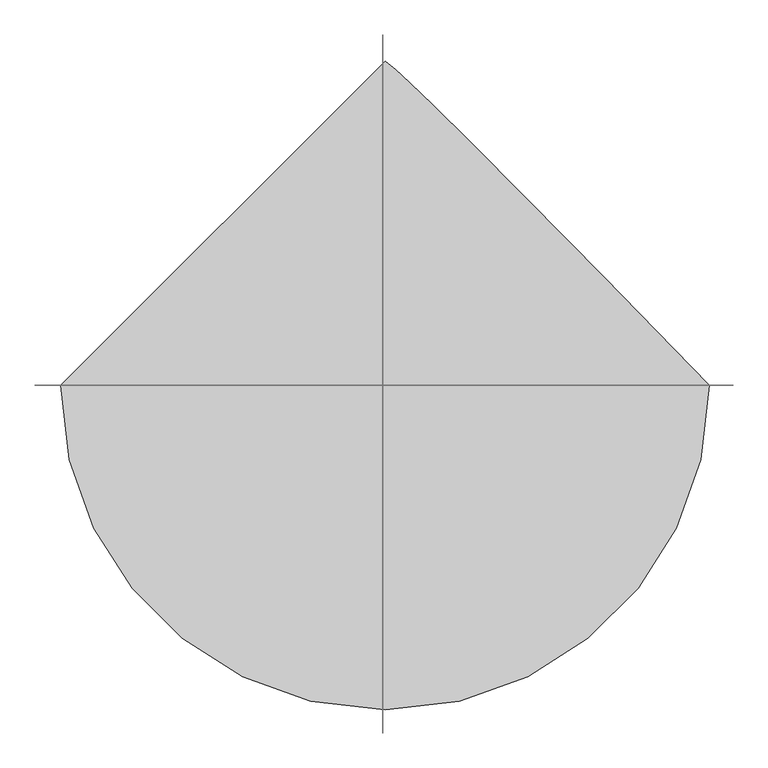
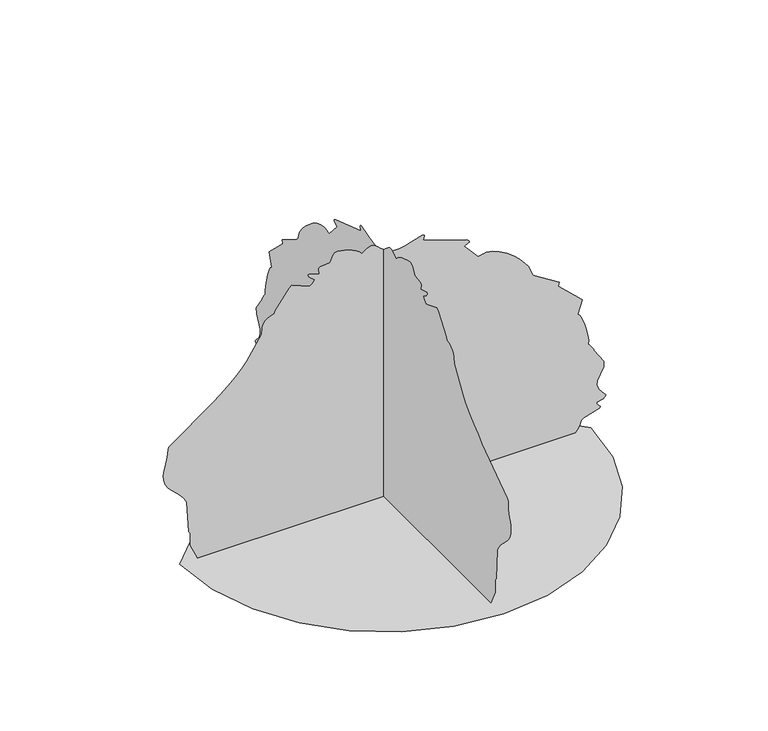
"""IFC4 building model written with IfcOpenShell, lengths in millimetres: proxy geometry, holly 26750 : holly 26750."""

import ifcopenshell
import ifcopenshell.guid

model = None  # the IFC model being written
_history = None  # IfcOwnerHistory: only IFC2X3 demands one
_inside = {}  # id of a spatial element -> (the spatial element, [elements in it])
_under = {}  # id of a project, library or spatial element -> (it, [spatial elements below it])
_declared = {}  # id of a project -> (the project, [libraries it declares])
_typed = {}  # id of a type object -> (the type object, [elements of that type])
_made_of = {}  # id of a material, layer set ... -> (it, [elements and type objects made of it])


def new_model(schema):
    """Start an empty IFC model of exactly this schema.

    Asked for "IFC4X3", IfcOpenShell would pick the latest addendum, in which some entities
    have other attributes; the version numbers below select the first issue.
    IFC2X3 requires an IfcOwnerHistory on every rooted entity: one is made here for all.
    """
    global model, _history
    if schema == "IFC4X3":
        model = ifcopenshell.file(schema_version=(4, 3, 0, 0))
    else:
        model = ifcopenshell.file(schema=schema)
    _inside.clear()
    _under.clear()
    _declared.clear()
    _typed.clear()
    _made_of.clear()
    _history = None
    if model.schema == "IFC2X3":
        org = make("IfcOrganization", Name="unknown")
        user = make(
            "IfcPersonAndOrganization",
            ThePerson=make("IfcPerson", FamilyName="unknown"),
            TheOrganization=org,
        )
        app = make(
            "IfcApplication",
            ApplicationDeveloper=org,
            Version="unknown",
            ApplicationFullName="unknown",
            ApplicationIdentifier="unknown",
        )
        _history = make(
            "IfcOwnerHistory",
            OwningUser=user,
            OwningApplication=app,
            ChangeAction="ADDED",
            CreationDate=0,
        )
    return model


def make(cls, **values):
    """One entity of the class cls with the attributes given. An attribute that is None is left unset."""
    return model.create_entity(
        cls, **{name: value for name, value in values.items() if value is not None}
    )


def rooted(cls, **values):
    """An entity with a GlobalId (a new one), such as an element, a storey or a relation."""
    return make(cls, GlobalId=ifcopenshell.guid.new(), OwnerHistory=_history, **values)


def si_unit(unit_type, name, prefix=None):
    """IfcSIUnit, for example si_unit("LENGTHUNIT", "METRE", prefix="MILLI")."""
    return make("IfcSIUnit", UnitType=unit_type, Prefix=prefix, Name=name)


def assignment(units):
    """IfcUnitAssignment: the units of a project."""
    return None if units is None else make("IfcUnitAssignment", Units=units)


def point(xyz):
    """IfcCartesianPoint."""
    return None if xyz is None else make("IfcCartesianPoint", Coordinates=xyz)


def direction(xyz):
    """IfcDirection."""
    return None if xyz is None else make("IfcDirection", DirectionRatios=xyz)


def frame(location, z_axis=None, x_axis=None):
    """IfcAxis2Placement3D, a coordinate frame: its origin and axes. An axis left out is left unset."""
    return make(
        "IfcAxis2Placement3D",
        Location=point(location),
        Axis=direction(z_axis),
        RefDirection=direction(x_axis),
    )


def origin():
    """The frame at (0, 0, 0) with its axes left unset."""
    return frame((0.0, 0.0, 0.0))


def place(relative_to, where):
    """IfcLocalPlacement: puts the frame where relative to a parent placement (None: the world)."""
    return make(
        "IfcLocalPlacement", PlacementRelTo=relative_to, RelativePlacement=where
    )


def context(
    kind, dimensions, precision=None, world=None, true_north=None, identifier=None
):
    """IfcGeometricRepresentationContext, for example the 3D "Model" context."""
    return make(
        "IfcGeometricRepresentationContext",
        ContextIdentifier=identifier,
        ContextType=kind,
        CoordinateSpaceDimension=dimensions,
        Precision=precision,
        WorldCoordinateSystem=world,
        TrueNorth=true_north,
    )


def project(units=None, contexts=None):
    """IfcProject with its units and contexts."""
    return rooted(
        "IfcProject",
        Name="project",
        RepresentationContexts=contexts,
        UnitsInContext=assignment(units),
    )


def spatial(cls, under=None, at=None, **own):
    """A site, building, storey or space (cls), placed at a placement, below another one or the project."""
    s = rooted(cls, ObjectPlacement=at, **own)
    if under is not None:
        _under.setdefault(under.id(), (under, []))[1].append(s)
    return s


def point_list(points):
    """IfcCartesianPointList2D or 3D."""
    cls = (
        "IfcCartesianPointList2D" if len(points[0]) == 2 else "IfcCartesianPointList3D"
    )
    return make(cls, CoordList=points)


def triangles(points, corners, closed=None, point_numbers=None):
    """IfcTriangulatedFaceSet: each triangle names its three corners, points numbered from 1."""
    return make(
        "IfcTriangulatedFaceSet",
        Coordinates=point_list(points),
        Closed=closed,
        CoordIndex=corners,
        PnIndex=point_numbers,
    )


def shape(context_of_items, identifier, shape_type, items):
    """IfcShapeRepresentation: the items that make up one representation, for example the "Body"."""
    return make(
        "IfcShapeRepresentation",
        ContextOfItems=context_of_items,
        RepresentationIdentifier=identifier,
        RepresentationType=shape_type,
        Items=items,
    )


def source(mapping_origin, context_of_items, identifier, shape_type, items):
    """IfcRepresentationMap: a shape defined once, which mapped items show again and again."""
    return make(
        "IfcRepresentationMap",
        MappingOrigin=mapping_origin,
        MappedRepresentation=shape(context_of_items, identifier, shape_type, items),
    )


def transform(
    local_origin,
    x_axis=None,
    y_axis=None,
    z_axis=None,
    scale=None,
    scale2=None,
    scale3=None,
    uniform=True,
):
    """IfcCartesianTransformationOperator3D, or its non-uniform kind. x_axis, y_axis, z_axis: its Axis1, 2, 3."""
    if uniform:
        return make(
            "IfcCartesianTransformationOperator3D",
            Axis1=direction(x_axis),
            Axis2=direction(y_axis),
            LocalOrigin=point(local_origin),
            Scale=scale,
            Axis3=direction(z_axis),
        )
    return make(
        "IfcCartesianTransformationOperator3DnonUniform",
        Axis1=direction(x_axis),
        Axis2=direction(y_axis),
        LocalOrigin=point(local_origin),
        Scale=scale,
        Axis3=direction(z_axis),
        Scale2=scale2,
        Scale3=scale3,
    )


def mapped(mapping_source, mapping_target):
    """IfcMappedItem: shows the shape of a source again, moved by a transform."""
    return make(
        "IfcMappedItem", MappingSource=mapping_source, MappingTarget=mapping_target
    )


def made_of(thing, what):
    """Note that an element or type object is made of a material, layer set ...; save() writes the relation."""
    if what is not None:
        _made_of.setdefault(what.id(), (what, []))[1].append(thing)
    return thing


def element(
    cls,
    number,
    at=None,
    inside=None,
    cuts=None,
    type_object=None,
    material=None,
    context=None,
    identifier="Body",
    shape_type=None,
    held_by="IfcProductDefinitionShape",
    body=None,
    shapes=None,
    **own,
):
    """One element of the class cls, such as IfcWall. Its Tag is "e" and its number.

    at: its placement. inside: the storey or other place that contains it. cuts: it is an
    opening in that element (IfcRelVoidsElement). A single representation is given by context,
    identifier, shape_type and body (its items); several are given by shapes. held_by: the class
    of the entity that holds the representations. save() writes the other relations.
    """
    e = rooted(cls, Tag="e%d" % number, ObjectPlacement=at, **own)
    if body is not None:
        shapes = [shape(context, identifier, shape_type, body)]
    if shapes is not None:
        e.Representation = make(held_by, Representations=shapes)
    if inside is not None:
        _inside.setdefault(inside.id(), (inside, []))[1].append(e)
    if cuts is not None:
        rooted(
            "IfcRelVoidsElement", RelatingBuildingElement=cuts, RelatedOpeningElement=e
        )
    if type_object is not None:
        _typed.setdefault(type_object.id(), (type_object, []))[1].append(e)
    return made_of(e, material)


def aggregate(whole, parts):
    """IfcRelAggregates: a whole, such as a stair, and the parts it consists of."""
    return rooted("IfcRelAggregates", RelatingObject=whole, RelatedObjects=parts)


def save(model, path):
    """Write the relations noted so far, then the file.

    IfcRelAggregates (storeys below a building ...), IfcRelContainedInSpatialStructure (elements
    in a storey), IfcRelDefinesByType, IfcRelAssociatesMaterial and IfcRelDeclares: one each for
    every whole, place, type object, material and project.
    """
    for whole, parts in _under.values():
        aggregate(whole, parts)
    for where, things in _inside.values():
        rooted(
            "IfcRelContainedInSpatialStructure",
            RelatedElements=things,
            RelatingStructure=where,
        )
    for kind, things in _typed.values():
        rooted("IfcRelDefinesByType", RelatedObjects=things, RelatingType=kind)
    for what, things in _made_of.values():
        rooted("IfcRelAssociatesMaterial", RelatedObjects=things, RelatingMaterial=what)
    for by, libraries in _declared.values():
        rooted("IfcRelDeclares", RelatingContext=by, RelatedDefinitions=libraries)
    model.write(path)


def entourage_c51d7213(model_context):
    return source(origin(), model_context, "Body", "Tessellation", [
        triangles([(-948.1489574, 0.0, 0.0001584), (-923.0842083, -217.2530545, 0.0001584), (-851.6949612, -416.7657311, 0.0001584), (-739.7012884, -592.8207553, 0.0001584), (-592.8207553, -739.7012884, 0.0001584), (-416.7657311, -851.6949612, 0.0001584), (-217.2530545, -923.0816648, 0.0001584), (4.14e-05, -948.1489574, 0.0001584), (217.2530545, -923.0842083, 0.0001584), (416.7657311, -851.6949612, 0.0001584), (592.8207553, -739.7012884, 0.0001584), (739.7012884, -592.8207553, 0.0001584), (851.6949612, -416.7657311, 0.0001584), (923.0816648, -217.2530545, 0.0001584), (948.1489574, 8.29e-05, 0.0001584), (640.0215443, 316.0623576, 0.0001584), (411.5917374, 548.7669763, 0.0001584), (249.5753185, 712.0026157, 0.0001584), (140.6913579, 819.6655935, 0.0001584), (71.6559369, 885.64972, 0.0001584), (29.1863771, 923.8462257, 0.0001584), (-0.0001243, 948.1489574, 0.0001584), (-7.5086714, -195.1763861, 1267.2389282), (-7.5086714, -179.2483067, 1263.2994884), (-7.5086714, -162.0304078, 1257.8307816), (-7.5086714, -144.4787539, 1250.7569401), (-7.5086714, -127.5514259, 1242.0092182), (-7.5086714, -112.2047518, 1231.5139286), (-7.5086714, -99.3960405, 1219.1973839), (-7.5086714, -96.3241623, 1220.6731659), (-7.5086714, -91.1522123, 1224.4323841), (-7.5086714, -84.5334848, 1229.4921043), (-7.5086714, -77.1194751, 1234.8564571), (-7.5086714, -69.5642495, 1239.5377121), (-7.5086714, -62.5195578, 1242.5399998), (-7.5086714, -56.6381899, 1242.880386), (-7.5086714, -48.1497636, 1241.0642178), (-7.5086714, -38.0075433, 1235.3112259), (-7.5086714, -26.6616175, 1226.6954727), (-7.5086714, -14.5605495, 1216.2942181), (-7.5086714, -2.1549868, 1205.1816696), (-7.5086714, 10.1063292, 1194.4323984), (-7.5086714, 21.7735642, 1185.1233009), (-7.5086714, 44.9310738, 1181.1406225), (-7.5086714, 71.2939859, 1182.9871668), (-7.5086714, 98.7844045, 1188.6996088), (-7.5086714, 125.3246087, 1196.3018337), (-7.5086714, 178.4657237, 1210.777331), (-7.5086714, 184.0044481, 1210.1194496), (-7.5086714, 186.6691655, 1206.9444254), (-7.5086714, 187.1967314, 1202.1768385), (-7.5086714, 182.6755321, 1185.5170269), (-7.5086714, 383.1462716, 1117.5161631), (-7.5086714, 393.1767277, 1109.7361147), (-7.5086714, 395.0157143, 1105.6136919), (-7.5086714, 393.8879488, 1102.1694254), (-7.5086714, 390.6062814, 1099.2180067), (-7.5086714, 372.1277581, 1088.6871088), (-7.5086714, 435.2772466, 1017.1175674), (-7.5086714, 437.7283324, 1017.437606), (-7.5086714, 442.2698793, 1018.3037596), (-7.5086714, 448.2439333, 1019.5610229), (-7.5086714, 454.9825481, 1021.0621668), (-7.5086714, 461.822792, 1022.6598164), (-7.5086714, 468.1067471, 1024.2016554), (-7.5086714, 473.166431, 1025.537693), (-7.5086714, 502.5059555, 1020.5592905), (-7.5086714, 534.2381756, 1007.0464525), (-7.5086714, 566.6435014, 987.1252121), (-7.5086714, 598.0048865, 962.9266891), (-7.5086714, 626.6103716, 936.5792421), (-7.5086714, 650.7352798, 910.2089767), (-7.5086714, 668.6702316, 885.9468676), (-7.5086714, 686.5644882, 838.1898262), (-7.5086714, 809.9704004, 760.305772), (-7.5086714, 805.7591022, 743.4655935), (-7.5086714, 915.2203714, 638.2130791), (-7.5086714, 894.1714382, 575.0635906), (-7.5086714, 903.617664, 567.5579078), (-7.5086714, 914.1053232, 547.8068604), (-7.5086714, 924.5625338, 519.9684434), (-7.5086714, 933.9198841, 488.2006877), (-7.5086714, 941.1080355, 456.6564285), (-7.5086714, 945.0552509, 429.4962041), (-7.5086714, 944.6894302, 410.8729222), (-7.5086714, 947.6840876, 408.4091191), (-7.5086714, 951.631303, 403.9311221), (-7.5086714, 956.0813948, 398.0789357), (-7.5086714, 960.5872971, 391.4952533), (-7.5086714, 964.7020895, 384.820152), (-7.5086714, 967.971076, 378.6987597), (-7.5086714, 969.9497343, 373.7711535), (-7.5086714, 1015.9974323, 304.568855), (-7.5086714, 1014.0136871, 276.7279126), (-7.5086714, 984.4354053, 218.9253907), (-7.5086714, 983.4092325, 198.3142941), (-7.5086714, 995.1541552, 172.0712739), (-7.5086714, 1024.6817133, 137.2212117), (-7.5086714, 1022.9417759, 130.8493623), (-7.5086714, 1018.3139334, 126.0055809), (-7.5086714, 1011.6743677, 122.4462869), (-7.5086714, 982.5811581, 116.1709614), (-7.5086714, 982.5024565, 110.3304839), (-7.5086714, 984.7630743, 105.408982), (-7.5086714, 999.0657623, 90.4069817), (-7.5086714, 999.4214092, 86.700867), (-7.5086714, 994.9103474, 81.6175654), (-7.5086714, 922.3882479, 60.3801172), (-7.5086714, 911.0090733, 53.020719), (-7.5086714, 909.9524517, 45.2163171), (-7.5086714, 907.5597198, 37.5411996), (-7.5086714, 904.0596428, 29.9740312), (-7.5086714, 899.6679777, 22.4928926), (-7.5086714, 894.6082575, 15.0766517), (-7.5086714, 889.1066311, 7.7034389), (-7.5086714, 883.3814718, 0.3517747), (-7.5086714, -857.0696331, 0.0), (-7.5086714, -890.8821041, 74.070715), (-7.5086714, -890.8821041, 133.011158), (-7.5086714, -897.8544256, 142.0888652), (-7.5086714, -906.9323599, 288.2569691), (-7.5086714, -918.2785423, 310.329568), (-7.5086714, -934.7885084, 330.547956), (-7.5086714, -954.1814381, 349.7579753), (-7.5086714, -974.171279, 368.8105187), (-7.5086714, -992.4846233, 388.5513923), (-7.5086714, -1006.8356369, 409.831525), (-7.5086714, -1014.945825, 433.5017735), (-7.5086714, -1016.3835279, 454.0351496), (-7.5086714, -1014.4251446, 473.0826061), (-7.5086714, -1010.2722731, 490.9768991), (-7.5086714, -1005.1338512, 508.0558711), (-7.5086714, -996.7289864, 541.0987307), (-7.5086714, -993.7038076, 576.6841312), (-7.5086714, -989.7007816, 586.0592494), (-7.5086714, -986.7239285, 589.1733035), (-7.5086714, -784.7202702, 733.315777), (-7.5086714, -753.8211388, 759.3609169), (-7.5086714, -719.0663561, 789.2566938), (-7.5086714, -684.3724709, 820.8568726), (-7.5086714, -653.6486195, 852.0099129), (-7.5086714, -630.8089525, 880.5697248), (-7.5086714, -562.4982239, 987.6459652), (-7.5086714, -559.6966144, 1020.7294109), (-7.5086714, -555.292232, 1034.4301735), (-7.5086714, -548.0761027, 1046.0812065), (-7.5086714, -537.4512789, 1055.5756851), (-7.5086714, -522.8132552, 1062.7994448), (-7.5086714, -503.5575265, 1067.6381756), (-7.5086714, -500.3495101, 1081.6894255), (-7.5086714, -435.3305863, 1167.4931997), (-7.5086714, -423.5678596, 1177.0969013), (-7.5086714, -339.3668581, 1143.4165443), (-7.5086714, -336.5372706, 1144.8643484), (-7.5086714, -333.0320704, 1147.7802315), (-7.5086714, -329.2195487, 1151.7172005), (-7.5086714, -318.3178522, 1168.6768484), (-7.5086714, -338.9502774, 1184.7296476), (-7.5086714, -344.6017857, 1191.1278763), (-7.5086714, -347.962191, 1197.2136967), (-7.5086714, -347.7869473, 1202.3572054), (-7.5086714, -343.1539816, 1204.0539042), (-7.5086714, -297.2663574, 1189.7283251), (-7.5086714, -299.3516952, 1212.9287258), (-7.5086714, -298.767483, 1216.5431128), (-7.5086714, -297.2663574, 1219.1973839), (-7.5086714, -292.6613332, 1221.3539383), (-7.5086714, -249.2443431, 1226.9900768), (-7.5086714, -246.747021, 1227.6175095), (-7.5086714, -231.2268564, 1258.3413609), (-7.5086714, -224.3381235, 1265.7124226), (-7.5086714, -216.7902557, 1269.9999516), (-7.5086714, -208.8568192, 1269.717992), (-202.6848849, -7.94e-05, 1267.2389282), (-186.7567873, -7.9e-05, 1263.2994884), (-169.5388885, -7.87e-05, 1257.8307816), (-151.9872436, -7.84e-05, 1250.7569401), (-135.0599247, -7.8e-05, 1242.0092182), (-119.7134959, -7.75e-05, 1231.5139286), (-106.9047846, -7.68e-05, 1219.1973839), (-103.8329063, -7.69e-05, 1220.6731659), (-98.6609655, -7.7e-05, 1224.4323841), (-92.0419745, -7.73e-05, 1229.4921043), (-84.6279739, -7.75e-05, 1234.8564571), (-77.0729936, -7.78e-05, 1239.5377121), (-70.0280521, -7.8e-05, 1242.5399998), (-64.1469339, -7.83e-05, 1242.880386), (-55.6582578, -7.75e-05, 1241.0642178), (-45.5160353, -7.69e-05, 1235.3112259), (-34.1701118, -7.64e-05, 1226.6954727), (-22.0691448, -7.6e-05, 1216.2942181), (-9.6635817, -7.56e-05, 1205.1816696), (2.5977342, -7.53e-05, 1194.4323984), (14.26497, -7.48e-05, 1185.1233009), (37.4223274, -7.46e-05, 1181.1406225), (63.7852418, -7.46e-05, 1182.9871668), (91.2759148, -7.49e-05, 1188.6996088), (117.816119, -7.54e-05, 1196.3018337), (170.9569705, -7.63e-05, 1210.777331), (176.4956949, -7.62e-05, 1210.1194496), (179.1604124, -7.6e-05, 1206.9444254), (179.6879783, -7.57e-05, 1202.1768385), (175.1670333, -7.48e-05, 1185.5170269), (375.6380453, -7.06e-05, 1117.5161631), (385.6685014, -7.03e-05, 1109.7361147), (387.5074516, -7.02e-05, 1105.6136919), (386.3797225, -7e-05, 1102.1694254), (383.0980187, -6.98e-05, 1099.2180067), (364.6195318, -6.91e-05, 1088.6871088), (427.7690203, -6.48e-05, 1017.1175674), (430.2201061, -6.48e-05, 1017.437606), (434.7616167, -6.49e-05, 1018.3037596), (440.735707, -6.5e-05, 1019.5610229), (447.4743218, -6.5e-05, 1021.0621668), (454.3145293, -6.51e-05, 1022.6598164), (460.5984844, -6.52e-05, 1024.2016554), (465.6581683, -6.53e-05, 1025.537693), (494.9977292, -6.5e-05, 1020.5592905), (526.7299493, -6.42e-05, 1007.0464525), (559.1352751, -6.3e-05, 987.1252121), (590.4966239, -6.16e-05, 962.9266891), (619.0995655, -6e-05, 936.5792421), (643.2270172, -5.84e-05, 910.2089767), (661.161969, -5.7e-05, 885.9468676), (679.0537548, -5.41e-05, 838.1898262), (802.4621378, -4.95e-05, 760.305772), (798.2508396, -4.85e-05, 743.4655935), (907.7121815, -4.22e-05, 638.2156225), (886.6606321, -3.85e-05, 575.0635906), (896.1094013, -3.8e-05, 567.5579078), (906.5970606, -3.68e-05, 547.8068604), (917.0542711, -3.52e-05, 519.9684434), (926.4116215, -3.33e-05, 488.2006877), (933.5973021, -3.14e-05, 456.6564285), (937.5444448, -2.98e-05, 429.4962041), (937.1812403, -2.87e-05, 410.8729222), (940.1758976, -2.85e-05, 408.4091191), (944.1230404, -2.83e-05, 403.9311221), (948.5731321, -2.79e-05, 398.0789357), (953.0791071, -2.75e-05, 391.4952533), (957.1913561, -2.71e-05, 384.820152), (960.462886, -2.68e-05, 378.6987597), (962.4415443, -2.65e-05, 373.7711535), (1008.4891697, -2.23e-05, 304.568855), (1006.5054245, -2.07e-05, 276.7279126), (976.9271427, -1.72e-05, 218.9253907), (975.9009699, -1.6e-05, 198.3142941), (987.6459652, -1.44e-05, 172.0712739), (1017.1734507, -1.24e-05, 137.2212117), (1015.4335133, -1.2e-05, 130.8493623), (1010.8056707, -1.17e-05, 126.0058353), (1004.1661051, -1.15e-05, 122.4462869), (975.0729681, -1.11e-05, 116.1712157), (974.9941938, -1.11e-05, 110.3304839), (977.2548117, -1.08e-05, 105.408982), (991.5575724, -9.4e-06, 90.407236), (991.9131466, -9.3e-06, 86.700867), (987.4020847, -9.1e-06, 81.6175654), (914.8800579, -7.5e-06, 60.3801172), (903.5008106, -7.3e-06, 53.020719), (902.4441891, -7.5e-06, 45.2163171), (900.0515299, -7.5e-06, 37.5411996), (896.5488367, -7.3e-06, 29.9740312), (892.1597151, -6.9e-06, 22.4929448), (887.1000675, -6.5e-06, 15.0767278), (881.5984411, -6e-06, 7.7034894), (875.8732819, -5.5e-06, 0.3518408), (-864.5778957, -4.1e-06, 6.72e-05), (-898.3903667, -8.6e-06, 74.0709693), (-898.3903667, -1.21e-05, 133.011158), (-905.3626156, -1.26e-05, 142.0888652), (-914.4406225, -2.14e-05, 288.2569691), (-925.7893484, -2.27e-05, 310.3321115), (-942.296771, -2.39e-05, 330.547956), (-961.6897007, -2.5e-05, 349.7579753), (-981.6820124, -2.62e-05, 368.8105187), (-999.992886, -2.73e-05, 388.5513923), (-1014.3438995, -2.86e-05, 409.831525), (-1022.4540876, -3e-05, 433.5017735), (-1023.8917179, -3.12e-05, 454.0351496), (-1021.9334072, -3.24e-05, 473.0826061), (-1017.7805357, -3.34e-05, 490.9768991), (-1012.6421139, -3.45e-05, 508.0558711), (-1004.237249, -3.64e-05, 541.0987307), (-1001.2146137, -3.86e-05, 576.6841312), (-997.2090443, -3.92e-05, 586.0592494), (-994.2347345, -3.94e-05, 589.1733035), (-792.2285328, -4.83e-05, 733.315777), (-761.3294014, -5.01e-05, 759.3609169), (-726.5746187, -5.21e-05, 789.2566938), (-691.8807335, -5.41e-05, 820.8568726), (-661.1568821, -5.59e-05, 852.0099129), (-638.3172152, -5.74e-05, 880.5697248), (-570.0064502, -6.3e-05, 987.6459652), (-567.2048407, -6.5e-05, 1020.7294109), (-562.8004947, -6.58e-05, 1034.4301735), (-555.584329, -6.65e-05, 1046.0812065), (-544.9595052, -6.71e-05, 1055.5756851), (-530.3215178, -6.75e-05, 1062.7994448), (-511.0682962, -6.78e-05, 1067.6381756), (-507.8577364, -6.87e-05, 1081.6894255), (-442.8413561, -7.38e-05, 1167.4931997), (-431.0760859, -7.43e-05, 1177.0969013), (-346.8750844, -7.23e-05, 1143.4165443), (-344.0455333, -7.24e-05, 1144.8643484), (-340.540333, -7.26e-05, 1147.7802315), (-336.727775, -7.28e-05, 1151.7172005), (-325.8261148, -7.38e-05, 1168.6768484), (-346.4585401, -7.48e-05, 1184.7296476), (-352.110012, -7.51e-05, 1191.1278763), (-355.4704536, -7.55e-05, 1197.2136967), (-355.2951736, -7.58e-05, 1202.3572054), (-350.6622442, -7.57e-05, 1204.0539042), (-304.7771271, -7.51e-05, 1189.7283251), (-306.8599397, -7.63e-05, 1212.9287258), (-306.2757457, -7.65e-05, 1216.5431128), (-304.7771271, -7.68e-05, 1219.1973839), (-300.1695595, -7.68e-05, 1221.3539383), (-256.7533506, -7.73e-05, 1226.9900768), (-254.2565372, -7.74e-05, 1227.6175095), (-238.7353552, -7.86e-05, 1258.3413609), (-231.8468767, -7.9e-05, 1265.7124226), (-224.2990089, -7.94e-05, 1269.9999516), (-216.3655724, -7.99e-05, 1269.717992)], [[21, 22, 1], [20, 21, 1], [19, 20, 1], [18, 19, 1], [17, 18, 1], [17, 1, 2], [17, 2, 3], [17, 3, 4], [16, 17, 4], [16, 4, 5], [16, 5, 6], [16, 6, 7], [16, 7, 8], [16, 8, 9], [16, 9, 10], [16, 10, 11], [16, 11, 12], [15, 16, 12], [14, 15, 12], [13, 14, 12], [74, 75, 76], [160, 161, 162], [116, 117, 118], [116, 118, 119], [76, 77, 78], [159, 160, 162], [158, 159, 162], [157, 158, 162], [157, 162, 163], [151, 152, 153], [115, 116, 119], [114, 115, 119], [113, 114, 119], [112, 113, 119], [111, 112, 119], [110, 111, 119], [109, 110, 119], [97, 98, 99], [97, 99, 100], [97, 100, 101], [97, 101, 102], [109, 119, 120], [109, 120, 121], [109, 121, 122], [105, 106, 107], [104, 105, 107], [104, 107, 108], [103, 104, 108], [150, 151, 153], [149, 150, 153], [48, 49, 50], [48, 50, 51], [48, 51, 52], [47, 48, 52], [109, 122, 123], [54, 55, 56], [54, 56, 57], [53, 54, 57], [53, 57, 58], [52, 53, 58], [108, 109, 123], [102, 103, 108], [92, 93, 94], [92, 94, 95], [96, 97, 102], [96, 102, 108], [96, 108, 123], [95, 96, 123], [92, 95, 123], [91, 92, 123], [90, 91, 123], [89, 90, 123], [88, 89, 123], [87, 88, 123], [86, 87, 123], [85, 86, 123], [84, 85, 123], [83, 84, 123], [82, 83, 123], [81, 82, 123], [80, 81, 123], [79, 80, 123], [78, 79, 123], [76, 78, 123], [74, 76, 123], [73, 74, 123], [72, 73, 123], [71, 72, 123], [70, 71, 123], [69, 70, 123], [68, 69, 123], [67, 68, 123], [66, 67, 123], [65, 66, 123], [64, 65, 123], [63, 64, 123], [62, 63, 123], [61, 62, 123], [60, 61, 123], [59, 60, 123], [58, 59, 123], [52, 58, 123], [47, 52, 123], [46, 47, 123], [45, 46, 123], [44, 45, 123], [43, 44, 123], [42, 43, 123], [41, 42, 123], [40, 41, 123], [39, 40, 123], [38, 39, 123], [37, 38, 123], [36, 37, 123], [35, 36, 123], [34, 35, 123], [33, 34, 123], [32, 33, 123], [31, 32, 123], [30, 31, 123], [29, 30, 123], [29, 123, 124], [28, 29, 124], [27, 28, 124], [26, 27, 124], [25, 26, 124], [24, 25, 124], [23, 24, 124], [173, 23, 124], [173, 124, 125], [173, 125, 126], [165, 166, 167], [164, 165, 167], [163, 164, 167], [163, 167, 168], [171, 172, 173], [170, 171, 173], [169, 170, 173], [169, 173, 126], [168, 169, 126], [168, 126, 127], [168, 127, 128], [168, 128, 129], [168, 129, 130], [168, 130, 131], [168, 131, 132], [145, 146, 147], [145, 147, 148], [144, 145, 148], [144, 148, 149], [143, 144, 149], [143, 149, 153], [142, 143, 153], [134, 135, 136], [133, 134, 136], [133, 136, 137], [132, 133, 137], [142, 153, 154], [156, 157, 163], [156, 163, 168], [141, 142, 154], [132, 137, 138], [132, 138, 139], [141, 154, 155], [140, 141, 155], [155, 156, 168], [155, 168, 132], [140, 155, 132], [140, 132, 139], [225, 226, 227], [311, 312, 313], [267, 268, 269], [267, 269, 270], [227, 228, 229], [310, 311, 313], [309, 310, 313], [308, 309, 313], [308, 313, 314], [302, 303, 304], [266, 267, 270], [265, 266, 270], [264, 265, 270], [263, 264, 270], [262, 263, 270], [261, 262, 270], [260, 261, 270], [248, 249, 250], [248, 250, 251], [248, 251, 252], [248, 252, 253], [260, 270, 271], [260, 271, 272], [260, 272, 273], [256, 257, 258], [255, 256, 258], [255, 258, 259], [254, 255, 259], [301, 302, 304], [300, 301, 304], [199, 200, 201], [199, 201, 202], [199, 202, 203], [198, 199, 203], [260, 273, 274], [205, 206, 207], [205, 207, 208], [204, 205, 208], [204, 208, 209], [203, 204, 209], [259, 260, 274], [253, 254, 259], [243, 244, 245], [243, 245, 246], [247, 248, 253], [247, 253, 259], [247, 259, 274], [246, 247, 274], [243, 246, 274], [242, 243, 274], [241, 242, 274], [240, 241, 274], [239, 240, 274], [238, 239, 274], [237, 238, 274], [236, 237, 274], [235, 236, 274], [234, 235, 274], [233, 234, 274], [232, 233, 274], [231, 232, 274], [230, 231, 274], [229, 230, 274], [227, 229, 274], [225, 227, 274], [224, 225, 274], [223, 224, 274], [222, 223, 274], [221, 222, 274], [220, 221, 274], [219, 220, 274], [218, 219, 274], [217, 218, 274], [216, 217, 274], [215, 216, 274], [214, 215, 274], [213, 214, 274], [212, 213, 274], [211, 212, 274], [210, 211, 274], [209, 210, 274], [203, 209, 274], [198, 203, 274], [197, 198, 274], [196, 197, 274], [195, 196, 274], [194, 195, 274], [193, 194, 274], [192, 193, 274], [191, 192, 274], [190, 191, 274], [189, 190, 274], [188, 189, 274], [187, 188, 274], [186, 187, 274], [185, 186, 274], [184, 185, 274], [183, 184, 274], [182, 183, 274], [181, 182, 274], [180, 181, 274], [180, 274, 275], [179, 180, 275], [178, 179, 275], [177, 178, 275], [176, 177, 275], [175, 176, 275], [174, 175, 275], [324, 174, 275], [324, 275, 276], [324, 276, 277], [316, 317, 318], [315, 316, 318], [314, 315, 318], [314, 318, 319], [322, 323, 324], [321, 322, 324], [320, 321, 324], [320, 324, 277], [319, 320, 277], [319, 277, 278], [319, 278, 279], [319, 279, 280], [319, 280, 281], [319, 281, 282], [319, 282, 283], [296, 297, 298], [296, 298, 299], [295, 296, 299], [295, 299, 300], [294, 295, 300], [294, 300, 304], [293, 294, 304], [285, 286, 287], [284, 285, 287], [284, 287, 288], [283, 284, 288], [293, 304, 305], [307, 308, 314], [307, 314, 319], [292, 293, 305], [283, 288, 289], [283, 289, 290], [292, 305, 306], [291, 292, 306], [306, 307, 319], [306, 319, 283], [291, 306, 283], [291, 283, 290]], closed=False),
    ])


if __name__ == "__main__":
    model = new_model("IFC4")
    model_context = context("Model", 3, world=origin())
    ifc_project = project(units=[si_unit("LENGTHUNIT", "METRE", prefix="MILLI")], contexts=[model_context])
    site = spatial("IfcSite", under=ifc_project)
    building = spatial("IfcBuilding", under=site)
    placement = place(None, origin())
    entourage_shape = entourage_c51d7213(model_context)
    element("IfcBuildingElementProxy", 1, Name="holly 26750 : holly 26750", ObjectType="holly 26750 : holly 26750", at=placement, inside=building, context=model_context, shape_type="MappedRepresentation", body=[
        mapped(entourage_shape, transform((0.0, 0.0, 0.0), x_axis=(1.0, 0.0, 0.0), y_axis=(0.0, 1.0, 0.0), z_axis=(0.0, 0.0, 1.0))),
    ])
    save(model, "model.ifc")

# Revit data of these elements
# Type "holly 26750 : holly 26750"
#   built-in parameter 1005195 = "RPC-16-FVGN-EMQ0-7PXJ-Q000-ST1L-LVER-AU"
#   Height = 0
